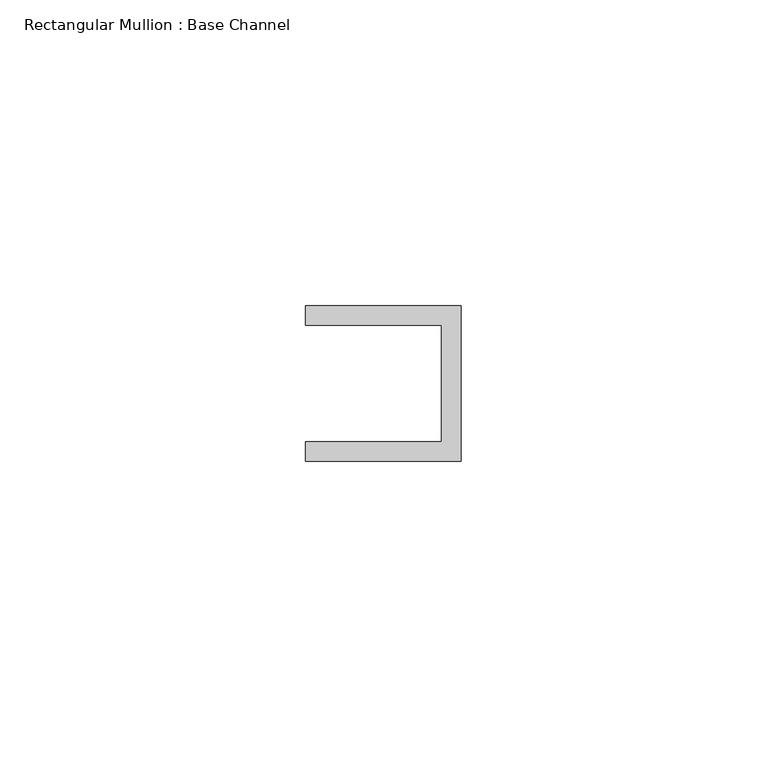
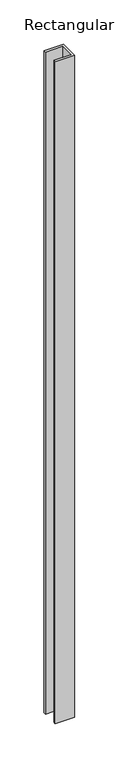
"""IFC4 building model written with IfcOpenShell, lengths in millimetres: member geometry, Rectangular Mullion : Base Channel."""

from ifc_helpers import new_model, si_unit, frame, origin, place, context, project, spatial, polyline, outline, extrude, source, transform, mapped, element, save


def rectangular_mullion_base_channel_c86233e4(model_context):
    return source(origin(), model_context, "Body", "SweptSolid", [
        extrude(outline(polyline([(0.0, -12.7), (-25.4, -12.7), (-25.4, -9.525), (-3.175, -9.525), (-3.175, 9.525), (-25.4, 9.525), (-25.4, 12.7), (0.0, 12.7), (0.0, -12.7)])), frame((0.0, 0.0, -914.4000002), z_axis=(0.0, 0.0, 1.0), x_axis=(1.0, 0.0, 0.0)), (0.0, 0.0, 1.0), 914.4000002),
    ])


if __name__ == "__main__":
    model = new_model("IFC4")
    model_context = context("Model", 3, world=origin())
    ifc_project = project(units=[si_unit("LENGTHUNIT", "METRE", prefix="MILLI")], contexts=[model_context])
    site = spatial("IfcSite", under=ifc_project)
    building = spatial("IfcBuilding", under=site)
    placement = place(None, origin())
    rectangular_mullion_base_channel_shape = rectangular_mullion_base_channel_c86233e4(model_context)
    element("IfcMember", 1, ObjectType="Rectangular Mullion : Base Channel", at=placement, inside=building, context=model_context, shape_type="MappedRepresentation", body=[
        mapped(rectangular_mullion_base_channel_shape, transform((0.0, 0.0, 0.0), x_axis=(1.0, 0.0, 0.0), y_axis=(0.0, 1.0, 0.0), z_axis=(0.0, 0.0, 1.0))),
    ])
    save(model, "model.ifc")

# Revit data of these elements
# Type "Rectangular Mullion : Base Channel"
#   built-in parameter 1007322 = 0.0833333 (stored number, unit not read)
#   built-in parameter 1007321 = 0.0416667 (stored number, unit not read)
#   built-in parameter 1007320 = -0.03125 (stored number, unit not read)
# Element 1 (IfcMember, "Rectangular Mullion : Base Channel")
#   Materials on its faces: "ALUM"
# Materials
#   "ALUM": class "Generic", colour RGB 157 157 157, transparency 0, Cost = 0
